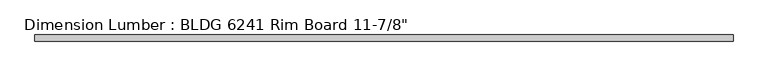
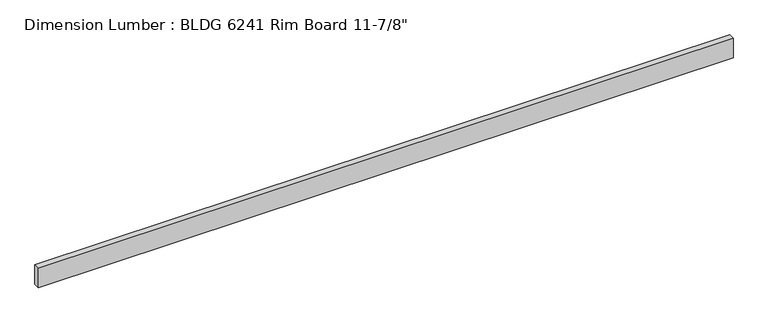
"""IFC4 building model written with IfcOpenShell, lengths in millimetres: beam geometry."""

from ifc_helpers import new_model, si_unit, frame, origin, place, context, project, spatial, polyline, outline, extrude, source, transform, mapped, element, save


def beam_ce0f0212(model_context):
    return source(origin(), model_context, "Body", "SweptSolid", [
        extrude(outline(polyline([(5041.9, 44.45), (5041.9, -44.45), (-5130.8, -44.45), (-5130.8, 44.45), (5041.9, 44.45)])), frame((0.0, 0.0, -150.8125), z_axis=(0.0, 0.0, 1.0), x_axis=(1.0, 0.0, 0.0)), (0.0, 0.0, 1.0), 301.625),
    ])


if __name__ == "__main__":
    model = new_model("IFC4")
    model_context = context("Model", 3, world=origin())
    ifc_project = project(units=[si_unit("LENGTHUNIT", "METRE", prefix="MILLI")], contexts=[model_context])
    site = spatial("IfcSite", under=ifc_project)
    building = spatial("IfcBuilding", under=site)
    placement = place(None, origin())
    beam_shape = beam_ce0f0212(model_context)
    element("IfcBeam", 1, ObjectType="Dimension Lumber : BLDG 6241 Rim Board 11-7/8\"", at=placement, inside=building, context=model_context, shape_type="MappedRepresentation", body=[
        mapped(beam_shape, transform((0.0, 0.0, 0.0), x_axis=(1.0, 0.0, 0.0), y_axis=(0.0, 1.0, 0.0), z_axis=(0.0, 0.0, 1.0))),
    ])
    save(model, "model.ifc")

# Revit data of these elements
# Type "Dimension Lumber : BLDG 6241 Rim Board 11-7/8\""
#   Assembly Code = "B10"
#   A = 0.273472 SF
#   Length [instance default] = 5' - 0"
#   b = 0' - 3 1/2"
#   d = 0' - 11 7/8"
#   Structural Material [instance default] = Softwood, Lumber
# Element 1 (IfcBeam, "Dimension Lumber : BLDG 6241 Rim Board 11-7/8\"")
#   Materials on its faces: "Softwood, Lumber"
# Materials
#   "Softwood, Lumber": class "Wood", colour RGB 223 192 134, transparency 0, Description = "Pinus Echinata", Cost = 0
